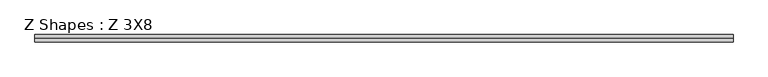
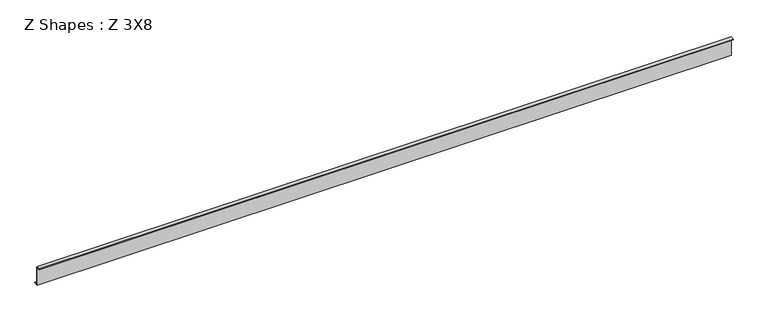
"""IFC4 building model written with IfcOpenShell, lengths in millimetres: beam geometry, Z Shapes : Z 3X8."""

from ifc_helpers import new_model, si_unit, frame, origin, place, context, project, spatial, polyline, outline, extrude, source, transform, mapped, element, save


def z_shapes_z_3x8_0fb0aa08(model_context):
    return source(origin(), model_context, "Body", "SweptSolid", [
        extrude(outline(polyline([(-57.2805719, 92.452825), (-57.2805719, 102.104825), (-19.1805719, 102.104825), (-19.1805719, -92.459175), (18.9194281, -92.459175), (18.9194281, -98.809175), (-27.1991352, -98.809175), (-27.1991352, 92.452825), (-57.2805719, 92.452825)])), frame((-3702.05, 0.0, 0.0), z_axis=(1.0, 0.0, 0.0), x_axis=(0.0, 1.0, 0.0)), (0.0, 0.0, 1.0), 7404.1),
    ])


if __name__ == "__main__":
    model = new_model("IFC4")
    model_context = context("Model", 3, world=origin())
    ifc_project = project(units=[si_unit("LENGTHUNIT", "METRE", prefix="MILLI")], contexts=[model_context])
    site = spatial("IfcSite", under=ifc_project)
    building = spatial("IfcBuilding", under=site)
    placement = place(None, origin())
    z_shapes_z_3x8_shape = z_shapes_z_3x8_0fb0aa08(model_context)
    element("IfcBeam", 1, ObjectType="Z Shapes : Z 3X8", at=placement, inside=building, context=model_context, shape_type="MappedRepresentation", body=[
        mapped(z_shapes_z_3x8_shape, transform((0.0, 0.0, 0.0), x_axis=(1.0, 0.0, 0.0), y_axis=(0.0, 1.0, 0.0), z_axis=(0.0, 0.0, 1.0))),
    ])
    save(model, "model.ifc")

# Revit data of these elements
# Type "Z Shapes : Z 3X8"
#   Section Name Key = "W12x26"
#   Assembly Code = "B10"
#   Width = 76.2 mm
#   Web Thickness = 5.842 mm
#   Web Fillet = 7.62 mm
#   Warping Constant = 163001.3 cm⁶
#   Torsional Moment of Inertia = 12.4869 cm⁴
#   Section Area = 7.65 in²
#   Plastic Modulus weak axis = 0.00472801 (stored number, unit not read)
#   Plastic Modulus strong axis = 0.0215278 (stored number, unit not read)
#   Perimeter = 15.0571 m²/m
#   Nominal Weight = 379.441 N/m
#   Moment of Inertia weak axis = 720.08 cm⁴
#   Moment of Inertia strong axis = 8491.12 cm⁴
#   Height = 184.912 mm
#   Flange Thickness = 9.652 mm
#   Elastic Modulus weak axis = 0.00309028 (stored number, unit not read)
#   Elastic Modulus strong axis = 0.0193287 (stored number, unit not read)
#   Centroid Vertical = 92.456 mm
#   Centroid Horizontal = 38.1 mm
#   Length [instance default] = 5' - 0"
#   Structural Material [instance default] = Steel ASTM A992
#   Principal Axes Angle = 0
# Element 1 (IfcBeam, "Z Shapes : Z 3X8")
#   Structural Material = none
# Materials
#   "Steel ASTM A992": class "Metal", colour RGB 189 187 185, transparency 0, Description = "Structural steel 50ksi", Cost = 0
